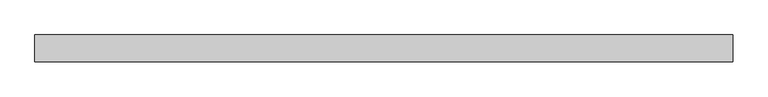
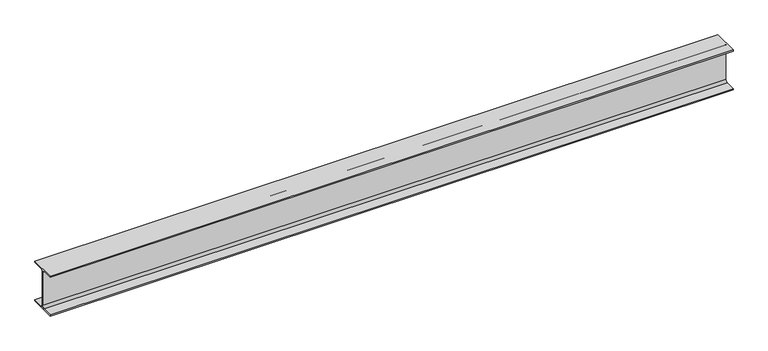
"""IFC4 building model written with IfcOpenShell, lengths in millimetres: beam geometry, 0912_Steel Framing_H-KSD3502 : H_SB_ASB_H-482x300x11x15."""

from ifc_helpers import new_model, si_unit, point, frame, frame_2d, origin, place, context, project, spatial, polyline, circle_curve, trimmed, segment, composite_curve, outline, extrude, source, transform, mapped, element, save


def beam_968140a5(model_context):
    return source(origin(), model_context, "Body", "SweptSolid", [
        extrude(outline(composite_curve([segment(polyline([(150.0, -226.0), (150.0, -241.0), (-150.0, -241.0), (-150.0, -226.0), (-31.5, -226.0)]), True, "CONTINUOUS"), segment(trimmed(circle_curve(frame_2d((-31.5, -200.0)), 26.0), [point((-31.5, -226.0))], [point((-5.5, -200.0))], True, "CARTESIAN"), True, "CONTINUOUS"), segment(polyline([(-5.5, -200.0), (-5.5, 200.0)]), True, "CONTINUOUS"), segment(trimmed(circle_curve(frame_2d((-31.5, 200.0)), 26.0), [point((-5.5, 200.0))], [point((-31.5, 226.0))], True, "CARTESIAN"), True, "CONTINUOUS"), segment(polyline([(-31.5, 226.0), (-150.0, 226.0), (-150.0, 241.0), (150.0, 241.0), (150.0, 226.0), (31.5, 226.0)]), True, "CONTINUOUS"), segment(trimmed(circle_curve(frame_2d((31.5, 200.0)), 26.0), [point((31.5, 226.0))], [point((5.5, 200.0))], True, "CARTESIAN"), True, "CONTINUOUS"), segment(polyline([(5.5, 200.0), (5.5, -200.0)]), True, "CONTINUOUS"), segment(trimmed(circle_curve(frame_2d((31.5, -200.0)), 26.0), [point((5.5, -200.0))], [point((31.5, -226.0))], True, "CARTESIAN"), True, "CONTINUOUS"), segment(polyline([(31.5, -226.0), (150.0, -226.0)]), True, "CONTINUOUS")], self_intersect=False)), frame((-3904.8, 0.0, 0.0), z_axis=(1.0, 0.0, 0.0), x_axis=(0.0, 1.0, 0.0)), (0.0, 0.0, 1.0), 7809.6),
    ])


if __name__ == "__main__":
    model = new_model("IFC4")
    model_context = context("Model", 3, world=origin())
    ifc_project = project(units=[si_unit("LENGTHUNIT", "METRE", prefix="MILLI")], contexts=[model_context])
    site = spatial("IfcSite", under=ifc_project)
    building = spatial("IfcBuilding", under=site)
    placement = place(None, origin())
    beam_shape = beam_968140a5(model_context)
    element("IfcBeam", 1, ObjectType="0912_Steel Framing_H-KSD3502 : H_SB_ASB_H-482x300x11x15", at=placement, inside=building, context=model_context, shape_type="MappedRepresentation", body=[
        mapped(beam_shape, transform((0.0, 0.0, 0.0), x_axis=(1.0, 0.0, 0.0), y_axis=(0.0, 1.0, 0.0), z_axis=(0.0, 0.0, 1.0))),
    ])
    save(model, "model.ifc")

# Revit data of these elements
# Type "0912_Steel Framing_H-KSD3502 : H_SB_ASB_H-482x300x11x15"
#   H_WM Code_1 = "S01AA001-00001 | Main Steel Structure Fabrication Work | Shelter/Building | Heavy Steel - Standard (Weight≥90KG/M) | Material: (   )"
#   H_WM Code_2 = "S03AA027-00001 | Main Steel Structure Erection Work | Shelter/Building | Heavy Steel (Weight≥90KG/M) | Material: (   )"
#   H_WM Code_3 = "S01AA010-00001 | Main Steel Structure Fabrication Work | Shelter/Building | Steel Painting/Coating | for Non-Fireproofed Steel Surface, Surface Preparation, Primer, Second & Final Coat | Material: (   )"
#   H_Q'ty Cal Type Tag = "SB-Q2"
#   Width = 30.0 cm
#   Web Thickness = 1.1 cm
#   Web Fillet = 2.6 cm
#   Warping Constant = 3680000.0 cm⁶
#   W = 0
#   Torsional Moment of Inertia = 88.2192 cm⁴
#   Section Area = 145.5 cm²
#   Plastic Modulus weak axis = 695.0 cm³
#   Plastic Modulus strong axis = 2790.0 cm³
#   Perimeter = 2.10 m²/m
#   Nominal Weight = 114.00 kgf/m
#   Moment of Inertia weak axis = 6760.00 cm⁴
#   Moment of Inertia strong axis = 60400.00 cm⁴
#   Height = 48.2 cm
#   Flange Thickness = 1.5 cm
#   Elastic Modulus weak axis = 451.0 cm³
#   Elastic Modulus strong axis = 2500.0 cm³
#   Centroid Vertical = 24.1 cm
#   Centroid Horizontal = 15.0 cm
#   Ix = 604000000
#   Length [instance default] = 1.5240 m
#   Zx = 2790000
#   b = 0.3000 m
#   h = 0.4820 m
#   r = 0.0260 m
#   s = 0.0110 m
#   t = 0.0150 m
#   A = 0.01455 m²
#   Structural Material [instance default] = Steel, 45-345
#   Assembly Code = ""
# Element 1 (IfcBeam, "0912_Steel Framing_H-KSD3502 : H_SB_ASB_H-482x300x11x15")
#   Structural Material = none
# Materials
#   "Steel, 45-345": class "Metal", colour RGB 189 187 185, transparency 0, Description = "Steel 345 MPa", Cost = 0
